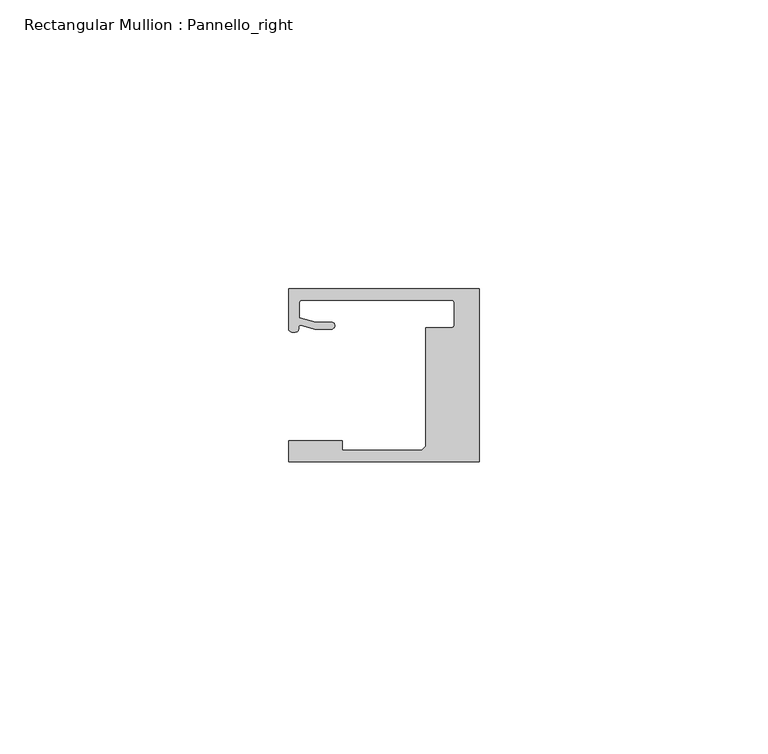
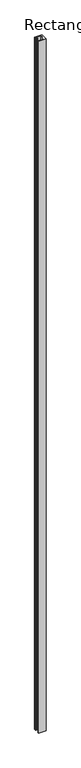
"""IFC4 building model written with IfcOpenShell, lengths in millimetres: member geometry, Rectangular Mullion : Pannello_right."""

from ifc_helpers import new_model, si_unit, frame, origin, place, context, project, spatial, polyline, circle_curve, source, transform, mapped, element, save
from ifc_brep_helpers import plane_surface, cylinder_surface, revolved_surface, extruded_surface, spline_curve, advanced_brep


def rectangular_mullion_pannello_right_c97d4869(model_context):
    return source(origin(), model_context, "Body", "AdvancedBrep", [
        advanced_brep(
        [(-33.0, -15.0, 0.0), (0.0, -15.0, 0.0), (0.0, 15.0, 0.0), (-33.0000135, 15.0, 0.0), (-33.0000135, 8.0000472, 0.0), (-30.9223017, 8.6490241, 0.0), (-28.4999305, 7.9999523, 0.0), (-25.59998, 7.9999523, 0.0), (-25.59998, 9.1999523, 0.0), (-28.3419477, 9.1999523, 0.0), (-31.19998, 9.9657591, 0.0), (-31.19998, 12.50001, 0.0), (-30.69998, 13.00001, 0.0), (-4.7999726, 13.00001, 0.0), (-4.2999726, 12.50001, 0.0), (-4.2999726, 8.7500595, 0.0), (-4.7999726, 8.2500595, 0.0), (-9.2999726, 8.2500595, 0.0), (-9.2999726, -12.2999849, 0.0), (-10.0000103, -13.0000004, 0.0), (-23.700041, -13.0000004, 0.0), (-23.700041, -11.3000004, 0.0), (-33.0, -11.3000004, 0.0), (-33.0, -15.0, -3248.9999865), (-33.0, -11.3000004, -3248.9999865), (-23.700041, -11.3000004, -3248.9999865), (-23.700041, -13.0000004, -3248.9999865), (-10.0000103, -13.0000004, -3248.9999865), (-9.2999726, -12.2999849, -3248.9999865), (-9.2999726, 8.2500595, -3248.9999865), (-4.7999726, 8.2500595, -3248.9999865), (-4.2999726, 8.7500595, -3248.9999865), (-4.2999726, 12.50001, -3248.9999865), (-4.7999726, 13.00001, -3248.9999865), (-30.69998, 13.00001, -3248.9999865), (-31.19998, 12.50001, -3248.9999865), (-31.19998, 9.9657591, -3248.9999865), (-28.3419477, 9.1999523, -3248.9999865), (-25.59998, 9.1999523, -3248.9999865), (-25.59998, 7.9999523, -3248.9999865), (-28.4999305, 7.9999523, -3248.9999865), (-30.9223017, 8.6490241, -3248.9999865), (-33.0000135, 8.0000472, -3248.9999865), (-33.0000135, 15.0, -3248.9999865), (0.0, 15.0, -3248.9999865), (0.0, -15.0, -3248.9999865)],
        [
            (0, 1),
            (1, 2),
            (2, 3),
            (3, 4),
            (4, 5, spline_curve(3, [(-33.0000135, 8.0000472, 0.0), (-33.0000135, 7.457047519, 0.0), (-32.262327879, 7.456527435, 0.0), (-31.357433266, 7.563996614, 0.0), (-31.305645054, 7.690065204, 0.0), (-31.298563602, 8.366228555, 0.0), (-31.312054066, 8.717747958, 0.0), (-30.9223017, 8.6490241, 0.0)], [4, 2, 2, 4], [0.0, 0.0027053965905959043, 0.0058611956533709, 0.007702013405570312])),
            (5, 6),
            (6, 7),
            (7, 8, circle_curve(frame((-25.59998, 8.5999523, 0.0), z_axis=(0.0, 0.0, 1.0), x_axis=(0.0, 1.0, 0.0)), 0.6)),
            (8, 9),
            (9, 10),
            (10, 11),
            (11, 12, circle_curve(frame((-30.69998, 12.50001, 0.0), z_axis=(0.0, 0.0, -1.0), x_axis=(0.0, 1.0, 0.0)), 0.5)),
            (12, 13),
            (13, 14, circle_curve(frame((-4.7999726, 12.50001, 0.0), z_axis=(0.0, 0.0, -1.0), x_axis=(1.0, 0.0, 0.0)), 0.5)),
            (14, 15),
            (15, 16, circle_curve(frame((-4.7999726, 8.7500595, 0.0), z_axis=(0.0, 0.0, -1.0), x_axis=(0.0, -1.0, 0.0)), 0.5)),
            (16, 17),
            (17, 18),
            (18, 19),
            (19, 20),
            (20, 21),
            (21, 22),
            (22, 0),
            (23, 24),
            (24, 25),
            (25, 26),
            (26, 27),
            (27, 28),
            (28, 29),
            (29, 30),
            (30, 31, circle_curve(frame((-4.7999726, 8.7500595, -3248.9999865), z_axis=(0.0, 0.0, 1.0), x_axis=(0.0, -1.0, 0.0)), 0.5)),
            (31, 32),
            (32, 33, circle_curve(frame((-4.7999726, 12.50001, -3248.9999865), z_axis=(0.0, 0.0, 1.0), x_axis=(1.0, 0.0, 0.0)), 0.5)),
            (33, 34),
            (34, 35, circle_curve(frame((-30.69998, 12.50001, -3248.9999865), z_axis=(0.0, 0.0, 1.0), x_axis=(0.0, 1.0, 0.0)), 0.5)),
            (35, 36),
            (36, 37),
            (37, 38),
            (38, 39, circle_curve(frame((-25.59998, 8.5999523, -3248.9999865), z_axis=(0.0, 0.0, -1.0), x_axis=(0.0, 1.0, 0.0)), 0.6)),
            (39, 40),
            (40, 41),
            (41, 42, spline_curve(3, [(-30.9223017, 8.6490241, -3248.9999865), (-31.312054066, 8.717747958, -3248.9999865), (-31.298563602, 8.366228555, -3248.9999865), (-31.305645054, 7.690065204, -3248.9999865), (-31.357433266, 7.563996614, -3248.9999865), (-32.262327879, 7.456527435, -3248.9999865), (-33.0000135, 7.457047519, -3248.9999865), (-33.0000135, 8.0000472, -3248.9999865)], [4, 2, 2, 4], [0.0, 0.001840817752199412, 0.004996616814974408, 0.007702013405570312])),
            (42, 43),
            (43, 44),
            (44, 45),
            (45, 23),
            (0, 23),
            (45, 1),
            (44, 2),
            (43, 3),
            (42, 4),
            (41, 5),
            (40, 6),
            (39, 7),
            (38, 8),
            (37, 9),
            (36, 10),
            (35, 11),
            (34, 12),
            (33, 13),
            (32, 14),
            (31, 15),
            (30, 16),
            (29, 17),
            (28, 18),
            (27, 19),
            (26, 20),
            (25, 21),
            (24, 22),
        ],
        [
            plane_surface(frame((0.0, -36.2491502, 0.0), z_axis=(0.0, 0.0, 1.0), x_axis=(-1.0, 0.0, 0.0))),
            plane_surface(frame((0.0, -36.2491502, -3248.9999865), z_axis=(0.0, 0.0, -1.0), x_axis=(-1.0, 0.0, 0.0))),
            plane_surface(frame((-33.0, -15.0, 0.0), z_axis=(0.0, -1.0, 0.0), x_axis=(0.0, 0.0, -1.0))),
            plane_surface(frame((0.0, -15.0, 0.0), z_axis=(1.0, 0.0, 0.0), x_axis=(0.0, 0.0, -1.0))),
            plane_surface(frame((0.0, 15.0, 0.0), z_axis=(0.0, 1.0, 0.0), x_axis=(0.0, 0.0, -1.0))),
            plane_surface(frame((-33.0000135, 15.0, 0.0), z_axis=(-1.0, 0.0, 0.0), x_axis=(0.0, 0.0, -1.0))),
            extruded_surface(spline_curve(3, [(-33.0000135, 8.0000472, -3248.9999865), (-33.0000135, 7.457047519, -3248.9999865), (-32.262327879, 7.456527435, -3248.9999865), (-31.357433266, 7.563996614, -3248.9999865), (-31.305645054, 7.690065204, -3248.9999865), (-31.298563602, 8.366228555, -3248.9999865), (-31.312054066, 8.717747958, -3248.9999865), (-30.9223017, 8.6490241, -3248.9999865)], [4, 2, 2, 4], [0.0, 0.0027053965905959043, 0.0058611956533709, 0.007702013405570312]), (0.0, 0.0, 3248.9999865), 3248.9999865),
            plane_surface(frame((-30.9223017, 8.6490241, 0.0), z_axis=(-0.2588188320019168, -0.965925883389178, 0.0), x_axis=(0.0, 0.0, -1.0))),
            plane_surface(frame((-28.4999305, 7.9999523, 0.0), z_axis=(0.0, -1.0, 0.0), x_axis=(0.0, 0.0, -1.0))),
            cylinder_surface(frame((-25.59998, 8.5999523, 0.0), z_axis=(0.0, 0.0, 1.0), x_axis=(0.0, 1.0, 0.0)), 0.6),
            plane_surface(frame((-25.59998, 9.1999523, 0.0), z_axis=(0.0, 1.0, 0.0), x_axis=(0.0, 0.0, -1.0))),
            plane_surface(frame((-28.3419477, 9.1999523, 0.0), z_axis=(0.2588188320428738, 0.9659258833782035, 0.0), x_axis=(0.0, 0.0, -1.0))),
            plane_surface(frame((-31.19998, 9.9657591, 0.0), z_axis=(1.0, 0.0, 0.0), x_axis=(0.0, 0.0, -1.0))),
            revolved_surface(polyline([(-30.69998, 13.00001, -3248.9999865), (-30.69998, 13.00001, 0.0)]), (-30.69998, 12.50001, 0.0), (0.0, 0.0, -1.0)),
            plane_surface(frame((-30.69998, 13.00001, 0.0), z_axis=(0.0, -1.0, 0.0), x_axis=(0.0, 0.0, -1.0))),
            revolved_surface(polyline([(-4.2999726, 12.50001, -3248.9999865), (-4.2999726, 12.50001, 0.0)]), (-4.7999726, 12.50001, 0.0), (0.0, 0.0, -1.0)),
            plane_surface(frame((-4.2999726, 12.50001, 0.0), z_axis=(-1.0, 0.0, 0.0), x_axis=(0.0, 0.0, -1.0))),
            revolved_surface(polyline([(-4.7999726, 8.2500595, -3248.9999865), (-4.7999726, 8.2500595, 0.0)]), (-4.7999726, 8.7500595, 0.0), (0.0, 0.0, -1.0)),
            plane_surface(frame((-4.7999726, 8.2500595, 0.0), z_axis=(0.0, 1.0, 0.0), x_axis=(0.0, 0.0, -1.0))),
            plane_surface(frame((-9.2999726, 8.2500595, 0.0), z_axis=(-1.0, 0.0, 0.0), x_axis=(0.0, 0.0, -1.0))),
            plane_surface(frame((-9.2999726, -12.2999849, 0.0), z_axis=(-0.7070955486278075, 0.7071180135668587, 0.0), x_axis=(0.0, 0.0, -1.0))),
            plane_surface(frame((-10.0000103, -13.0000004, 0.0), z_axis=(0.0, 1.0, 0.0), x_axis=(0.0, 0.0, -1.0))),
            plane_surface(frame((-23.700041, -13.0000004, 0.0), z_axis=(1.0, 0.0, 0.0), x_axis=(0.0, 0.0, -1.0))),
            plane_surface(frame((-23.700041, -11.3000004, 0.0), z_axis=(0.0, 1.0, 0.0), x_axis=(0.0, 0.0, -1.0))),
            plane_surface(frame((-33.0, -11.3000004, 0.0), z_axis=(-1.0, 0.0, 0.0), x_axis=(0.0, 0.0, -1.0))),
        ],
        [
            (0, [[1, 2, 3, 4, 5, 6, 7, 8, 9, 10, 11, 12, 13, 14, 15, 16, 17, 18, 19, 20, 21, 22, 23]]),
            (1, [[24, 25, 26, 27, 28, 29, 30, 31, 32, 33, 34, 35, 36, 37, 38, 39, 40, 41, 42, 43, 44, 45, 46]]),
            (2, [[-1, 47, -46, 48]]),
            (3, [[-2, -48, -45, 49]]),
            (4, [[-3, -49, -44, 50]]),
            (5, [[-4, -50, -43, 51]]),
            (6, [[-5, -51, -42, 52]]),
            (7, [[-6, -52, -41, 53]]),
            (8, [[-7, -53, -40, 54]]),
            (9, [[-8, -54, -39, 55]]),
            (10, [[-9, -55, -38, 56]]),
            (11, [[-10, -56, -37, 57]]),
            (12, [[-11, -57, -36, 58]]),
            (13, [[-12, -58, -35, 59]]),
            (14, [[-13, -59, -34, 60]]),
            (15, [[-14, -60, -33, 61]]),
            (16, [[-15, -61, -32, 62]]),
            (17, [[-16, -62, -31, 63]]),
            (18, [[-17, -63, -30, 64]]),
            (19, [[-18, -64, -29, 65]]),
            (20, [[-19, -65, -28, 66]]),
            (21, [[-20, -66, -27, 67]]),
            (22, [[-21, -67, -26, 68]]),
            (23, [[-22, -68, -25, 69]]),
            (24, [[-23, -69, -24, -47]]),
        ],
    ),
    ])


if __name__ == "__main__":
    model = new_model("IFC4")
    model_context = context("Model", 3, world=origin())
    ifc_project = project(units=[si_unit("LENGTHUNIT", "METRE", prefix="MILLI")], contexts=[model_context])
    site = spatial("IfcSite", under=ifc_project)
    building = spatial("IfcBuilding", under=site)
    placement = place(None, origin())
    rectangular_mullion_pannello_right_shape = rectangular_mullion_pannello_right_c97d4869(model_context)
    element("IfcMember", 1, ObjectType="Rectangular Mullion : Pannello_right", at=placement, inside=building, context=model_context, shape_type="MappedRepresentation", body=[
        mapped(rectangular_mullion_pannello_right_shape, transform((0.0, 0.0, 0.0), x_axis=(1.0, 0.0, 0.0), y_axis=(0.0, 1.0, 0.0), z_axis=(0.0, 0.0, 1.0))),
    ])
    save(model, "model.ifc")

# Revit data of these elements
# Type "Rectangular Mullion : Pannello_right"
#   built-in parameter 1007322 = 0.0984252 (stored number, unit not read)
#   built-in parameter 1007321 = 0.0305117 (stored number, unit not read)
#   built-in parameter 1007320 = 0 (stored number, unit not read)
